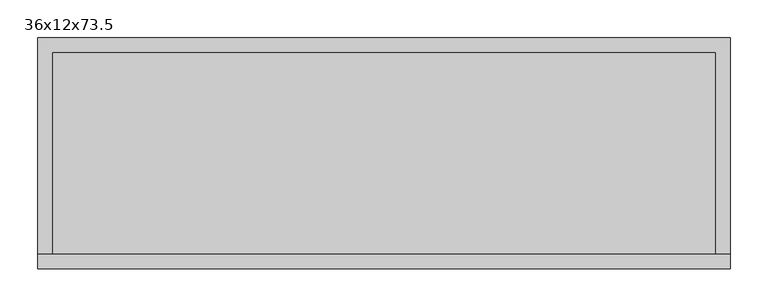
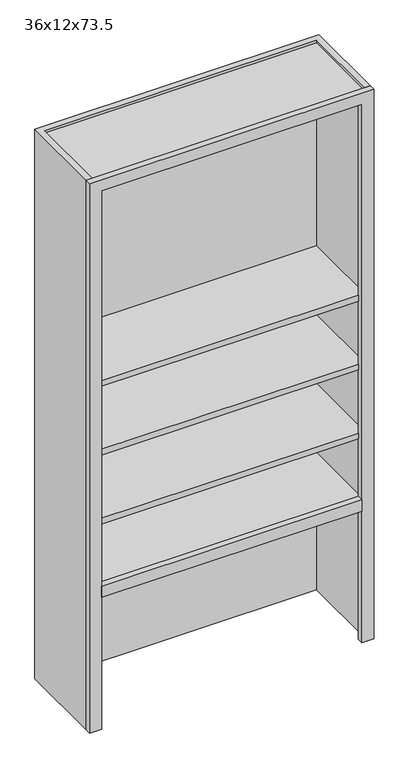
"""IFC4 building model written with IfcOpenShell, lengths in millimetres: furniture geometry, Bookcase-Merillat-Countertop : 36x12x73.5."""

from ifc_helpers import new_model, si_unit, frame, origin, place, context, project, spatial, polyline, outline, extrude, faceted_brep, source, transform, mapped, element, save


def furniture_36x12x73_5_dad68982(model_context):
    return source(origin(), model_context, "Body", "SolidModel", [
        extrude(outline(polyline([(-419.1, -133.35), (419.1, -133.35), (419.1, -152.4), (-419.1, -152.4), (-419.1, -133.35)])), frame((0.0, 0.0, 447.675), z_axis=(0.0, 0.0, 1.0), x_axis=(1.0, 0.0, 0.0)), (0.0, 0.0, 1.0), 38.1),
        extrude(outline(polyline([(-438.15, 133.35), (438.15, 133.35), (438.15, -133.35), (-438.15, -133.35), (-438.15, 133.35)])), frame((0.0, 0.0, 915.7607143), z_axis=(0.0, 0.0, 1.0), x_axis=(1.0, 0.0, 0.0)), (0.0, 0.0, 1.0), 19.3909952),
        extrude(outline(polyline([(-438.15, 133.35), (438.15, 133.35), (438.15, -133.35), (-438.15, -133.35), (-438.15, 133.35)])), frame((0.0, 0.0, 1149.4625763), z_axis=(0.0, 0.0, 1.0), x_axis=(1.0, 0.0, 0.0)), (0.0, 0.0, 1.0), 19.3909952),
        extrude(outline(polyline([(-438.15, 133.35), (438.15, 133.35), (438.15, -133.35), (-438.15, -133.35), (-438.15, 133.35)])), frame((0.0, 0.0, 681.5608645), z_axis=(0.0, 0.0, 1.0), x_axis=(1.0, 0.0, 0.0)), (0.0, 0.0, 1.0), 19.3909952),
        extrude(outline(polyline([(-438.15, 133.35), (438.15, 133.35), (438.15, -133.35), (-438.15, -133.35), (-438.15, 133.35)])), frame((0.0, 0.0, 447.675), z_axis=(0.0, 0.0, 1.0), x_axis=(1.0, 0.0, 0.0)), (0.0, 0.0, 1.0), 19.3909952),
        extrude(outline(polyline([(0.0, -457.2), (0.0, -419.1), (1828.8, -419.1), (1828.8, 419.1), (0.0, 419.1), (0.0, 457.2), (1866.9, 457.2), (1866.9, -457.2), (0.0, -457.2)])), frame((0.0, -152.4, 0.0), z_axis=(0.0, 1.0, 0.0), x_axis=(0.0, 0.0, 1.0)), (0.0, 0.0, 1.0), 19.05),
        faceted_brep([(-438.15, 133.35, 1857.6909423), (-438.15, -133.35, 1857.6909423), (438.15, -133.35, 1857.6909423), (438.15, 133.35, 1857.6909423), (-438.15, 133.35, 1866.9), (-438.15, -133.35, 1866.9), (438.15, -133.35, 1866.9), (438.15, 133.35, 1866.9), (-457.2, 152.4, 1866.9), (-457.2, -133.35, 1866.9), (457.2, -133.35, 1866.9), (457.2, 152.4, 1866.9), (-457.2, 152.4, 0.0), (457.2, 152.4, 0.0), (457.2, -133.35, 0.0), (438.15, -133.35, 0.0), (438.15, 133.35, 0.0), (-438.15, 133.35, 0.0), (-438.15, -133.35, 0.0), (-457.2, -133.35, 0.0), (-438.15, -133.35, 1847.5090048), (438.15, -133.35, 1847.5090048), (-438.15, 133.35, 1847.5090048), (438.15, 133.35, 1847.5090048)], [[[0, 1, 2, 3]], [[1, 0, 4, 5]], [[3, 2, 6, 7]], [[0, 3, 7, 4]], [[8, 9, 5, 4, 7, 6, 10, 11]], [[12, 13, 14, 15, 16, 17, 18, 19]], [[9, 8, 12, 19]], [[15, 14, 10, 6, 2, 1, 5, 9, 19, 18, 20, 21]], [[18, 17, 22, 20]], [[17, 16, 23, 22]], [[16, 15, 21, 23]], [[11, 10, 14, 13]], [[8, 11, 13, 12]], [[21, 20, 22, 23]]]),
    ])


if __name__ == "__main__":
    model = new_model("IFC4")
    model_context = context("Model", 3, world=origin())
    ifc_project = project(units=[si_unit("LENGTHUNIT", "METRE", prefix="MILLI")], contexts=[model_context])
    site = spatial("IfcSite", under=ifc_project)
    building = spatial("IfcBuilding", under=site)
    placement = place(None, origin())
    furniture_36x12x73_5_shape = furniture_36x12x73_5_dad68982(model_context)
    element("IfcFurniture", 1, ObjectType="Bookcase-Merillat-Countertop : 36x12x73.5", at=placement, inside=building, context=model_context, shape_type="MappedRepresentation", body=[
        mapped(furniture_36x12x73_5_shape, transform((0.0, 0.0, 0.0), x_axis=(1.0, 0.0, 0.0), y_axis=(0.0, 1.0, 0.0), z_axis=(0.0, 0.0, 1.0))),
    ])
    save(model, "model.ifc")

# Revit data of these elements
# Type "Bookcase-Merillat-Countertop : 36x12x73.5"
#   URL = "https://www.merillat.com/"
#   Product Page URL = "https://www.merillat.com/our-products/"
#   Product Documentation Link = "http://merillatbusiness.com/wp-content/uploads/2014/07/Merillat_Classic_Catalog.pdf"
#   Model = "BK1860"
#   Manufacturer = "Merillat"
#   Description = "Countertop Bookcase"
#   Construction Type = "Bookcase"
#   Assembly Code = "E2020200"
#   Width = 3' - 0"
#   Shelving Height = 0' - 9.21429"
#   Height = 6' - 1 1/2"
#   Depth = 1' - 0"
#   Default Elevation = 4' - 0"
#   Cabinet Shell = 0' - 0 3/4"
#   COBie.Type = no
#   Number of Shelves = 6
#   Shelving Material = Wood - Merillat - Pecan(1)
#   Bookcase Material = Wood - Merillat - Pecan(1)
# Element 1 (IfcFurniture, "Bookcase-Merillat-Countertop : 36x12x73.5")
#   Materials on its faces: "Wood - Merillat - Pecan(1)"
# Materials
#   "Wood - Merillat - Pecan(1)": class "Wood", colour RGB 108 67 43, transparency 0, Cost = 0
